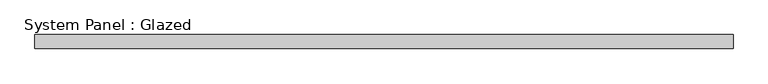
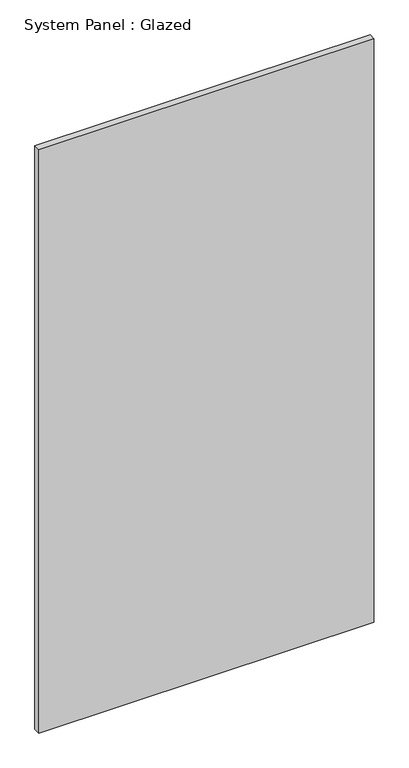
"""IFC4 building model written with IfcOpenShell, lengths in millimetres: plate geometry, System Panel : Glazed."""

from ifc_helpers import new_model, si_unit, origin, origin_with_axes, place, context, project, spatial, polyline, outline, extrude, source, transform, mapped, element, save


def system_panel_glazed_960e6087(model_context):
    return source(origin(), model_context, "Body", "SweptSolid", [
        extrude(outline(polyline([(625.0000001, 24.5), (-625.0000001, 24.5), (-625.0000001, 49.5), (625.0000001, 49.5), (625.0000001, 24.5)])), origin_with_axes(), (0.0, 0.0, 1.0), 2300.0),
    ])


if __name__ == "__main__":
    model = new_model("IFC4")
    model_context = context("Model", 3, world=origin())
    ifc_project = project(units=[si_unit("LENGTHUNIT", "METRE", prefix="MILLI")], contexts=[model_context])
    site = spatial("IfcSite", under=ifc_project)
    building = spatial("IfcBuilding", under=site)
    placement = place(None, origin())
    system_panel_glazed_shape = system_panel_glazed_960e6087(model_context)
    element("IfcPlate", 1, ObjectType="System Panel : Glazed", at=placement, inside=building, context=model_context, shape_type="MappedRepresentation", body=[
        mapped(system_panel_glazed_shape, transform((0.0, 0.0, 0.0), x_axis=(1.0, 0.0, 0.0), y_axis=(0.0, 1.0, 0.0), z_axis=(0.0, 0.0, 1.0))),
    ])
    save(model, "model.ifc")

# Revit data of these elements
# Type "System Panel : Glazed"
#   Construction Type Id = "GSP4R"
#   Analytic Construction = "1/8 in Pilkington single glazing"
#   Visual Light Transmittance = 0.9
#   Solar Heat Gain Coefficient = 0.86
#   Heat Transfer Coefficient (U) = 6.7069 W/(m²·K)
#   Define Thermal Properties by = 1
# Element 1 (IfcPlate, "System Panel : Glazed")
#   Materials on its faces: "Glass"
# Materials
#   "Glass": class "Glass", colour RGB 0 128 192, transparency 0.9, Description = "Soda Lime Glass", Cost = 0
